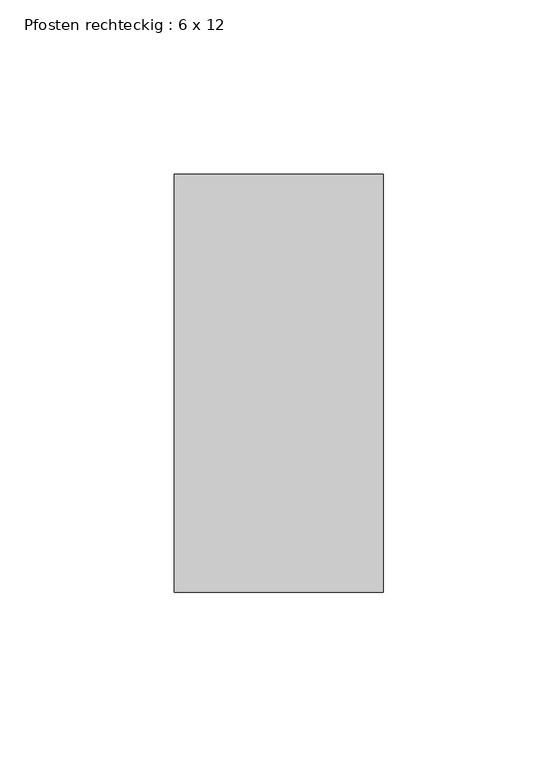
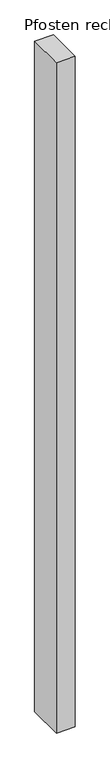
"""IFC4 building model written with IfcOpenShell, lengths in millimetres: member geometry, Pfosten rechteckig : 6 x 12."""

from ifc_helpers import new_model, si_unit, frame, origin, place, context, project, spatial, polyline, outline, extrude, source, transform, mapped, element, save


def pfosten_rechteckig_6_x_12_7d2c4df4(model_context):
    return source(origin(), model_context, "Body", "SweptSolid", [
        extrude(outline(polyline([(0.0, 60.0), (0.0, -60.0), (-60.0, -60.0), (-60.0, 60.0), (0.0, 60.0)])), frame((0.0, 0.0, -2267.088502), z_axis=(0.0, 0.0, 1.0), x_axis=(1.0, 0.0, 0.0)), (0.0, 0.0, 1.0), 2267.088502),
    ])


if __name__ == "__main__":
    model = new_model("IFC4")
    model_context = context("Model", 3, world=origin())
    ifc_project = project(units=[si_unit("LENGTHUNIT", "METRE", prefix="MILLI")], contexts=[model_context])
    site = spatial("IfcSite", under=ifc_project)
    building = spatial("IfcBuilding", under=site)
    placement = place(None, origin())
    pfosten_rechteckig_6_x_12_shape = pfosten_rechteckig_6_x_12_7d2c4df4(model_context)
    element("IfcMember", 1, ObjectType="Pfosten rechteckig : 6 x 12", at=placement, inside=building, context=model_context, shape_type="MappedRepresentation", body=[
        mapped(pfosten_rechteckig_6_x_12_shape, transform((0.0, 0.0, 0.0), x_axis=(1.0, 0.0, 0.0), y_axis=(0.0, 1.0, 0.0), z_axis=(0.0, 0.0, 1.0))),
    ])
    save(model, "model.ifc")

# Revit data of these elements
# Type "Pfosten rechteckig : 6 x 12"
#   built-in parameter 1007304 = 0.393701 (stored number, unit not read)
#   built-in parameter 1007301 = 0.0984252 (stored number, unit not read)
#   built-in parameter 1007300 = 0.0984252 (stored number, unit not read)
# Element 1 (IfcMember, "Pfosten rechteckig : 6 x 12")
#   Materials on its faces: "Metall - verzinkt"
# Materials
#   "Metall - verzinkt": class "Allgemeines", colour RGB 200 200 200, transparency 0, Cost = 0
